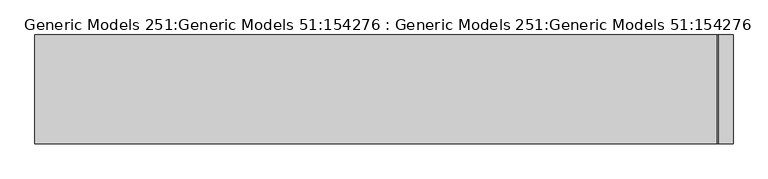
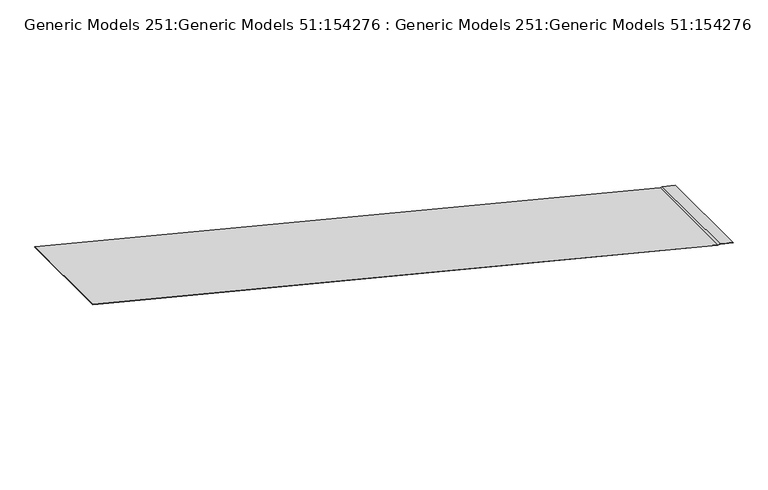
"""IFC4 building model written with IfcOpenShell, lengths in millimetres: proxy geometry, Generic Models 251:Generic Models 51:154276 : Generic Models 251:Generic Models 51:154276."""

from ifc_helpers import new_model, si_unit, frame, origin, place, context, project, spatial, polyline, outline, extrude, source, transform, mapped, element, save


def generic_models_251_generic_models_51_154276_generic_models_8951efe4(model_context):
    return source(origin(), model_context, "Body", "SweptSolid", [
        extrude(outline(polyline([(6461.6473906, 1757.0453218), (6459.9469315, 1750.6991219), (6936.3830169, -155.0452196), (6935.6129663, -155.2377322), (6459.1270288, 1750.7060178), (6460.8274879, 1757.0522176), (6450.963471, 1796.5082853), (6451.7335216, 1796.700798), (6461.6473906, 1757.0453218)])), frame((0.0, 5312.3878092, 0.0), z_axis=(0.0, 1.0, 0.0), x_axis=(0.0, 0.0, 1.0)), (0.0, 0.0, 1.0), 304.8),
    ])


if __name__ == "__main__":
    model = new_model("IFC4")
    model_context = context("Model", 3, world=origin())
    ifc_project = project(units=[si_unit("LENGTHUNIT", "METRE", prefix="MILLI")], contexts=[model_context])
    site = spatial("IfcSite", under=ifc_project)
    building = spatial("IfcBuilding", under=site)
    placement = place(None, origin())
    generic_models_251_generic_models_51_154276_generic_models_shape = generic_models_251_generic_models_51_154276_generic_models_8951efe4(model_context)
    element("IfcBuildingElementProxy", 1, Name="Generic Models 251:Generic Models 51:154276 : Generic Models 251:Generic Models 51:154276", ObjectType="Generic Models 251:Generic Models 51:154276 : Generic Models 251:Generic Models 51:154276", at=placement, inside=building, context=model_context, shape_type="MappedRepresentation", body=[
        mapped(generic_models_251_generic_models_51_154276_generic_models_shape, transform((0.0, 0.0, 0.0), x_axis=(1.0, 0.0, 0.0), y_axis=(0.0, 1.0, 0.0), z_axis=(0.0, 0.0, 1.0))),
    ])
    save(model, "model.ifc")

# Revit data of these elements
# Type "Generic Models 251:Generic Models 51:154276 : Generic Models 251:Generic Models 51:154276"
#   NameOverride = "Generic Models 251:Generic Models 51:154276"
#   ObjectTypeOverride = "Generic Models 251:Generic Models 51"
#   Reference = "Generic Models 51"
#   Category = "Generic Models"
#   Tag = "154276"
# Element 1 (IfcBuildingElementProxy, "Generic Models 251:Generic Models 51:154276 : Generic Models 251:Generic Models 51:154276")
#   Materials on its faces: "_(2) LAYERS NO. 30 ASTM D226 ASPHALT SATURATED ORGANIC FELT @ ROOF 21494"
# Materials
#   "_(2) LAYERS NO. 30 ASTM D226 ASPHALT SATURATED ORGANIC FELT @ ROOF 21494": class "Unassigned", colour RGB 67 154 161, transparency 0
